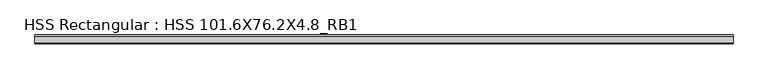
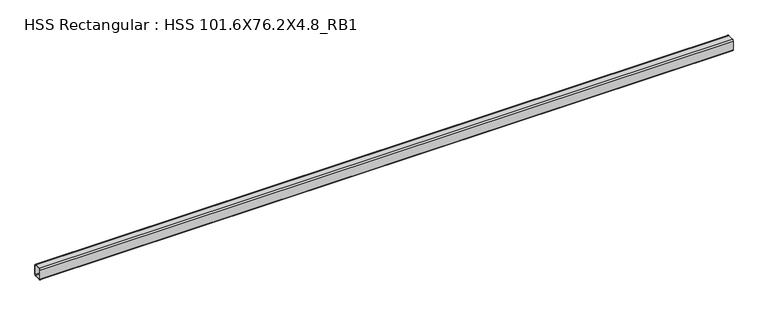
"""IFC4 building model written with IfcOpenShell, lengths in millimetres: beam geometry, HSS Rectangular : HSS 101.6X76.2X4.8_RB1."""

import ifcopenshell
import ifcopenshell.guid

model = None  # the IFC model being written
_history = None  # IfcOwnerHistory: only IFC2X3 demands one
_inside = {}  # id of a spatial element -> (the spatial element, [elements in it])
_under = {}  # id of a project, library or spatial element -> (it, [spatial elements below it])
_declared = {}  # id of a project -> (the project, [libraries it declares])
_typed = {}  # id of a type object -> (the type object, [elements of that type])
_made_of = {}  # id of a material, layer set ... -> (it, [elements and type objects made of it])


def new_model(schema):
    """Start an empty IFC model of exactly this schema.

    Asked for "IFC4X3", IfcOpenShell would pick the latest addendum, in which some entities
    have other attributes; the version numbers below select the first issue.
    IFC2X3 requires an IfcOwnerHistory on every rooted entity: one is made here for all.
    """
    global model, _history
    if schema == "IFC4X3":
        model = ifcopenshell.file(schema_version=(4, 3, 0, 0))
    else:
        model = ifcopenshell.file(schema=schema)
    _inside.clear()
    _under.clear()
    _declared.clear()
    _typed.clear()
    _made_of.clear()
    _history = None
    if model.schema == "IFC2X3":
        org = make("IfcOrganization", Name="unknown")
        user = make(
            "IfcPersonAndOrganization",
            ThePerson=make("IfcPerson", FamilyName="unknown"),
            TheOrganization=org,
        )
        app = make(
            "IfcApplication",
            ApplicationDeveloper=org,
            Version="unknown",
            ApplicationFullName="unknown",
            ApplicationIdentifier="unknown",
        )
        _history = make(
            "IfcOwnerHistory",
            OwningUser=user,
            OwningApplication=app,
            ChangeAction="ADDED",
            CreationDate=0,
        )
    return model


def make(cls, **values):
    """One entity of the class cls with the attributes given. An attribute that is None is left unset."""
    return model.create_entity(
        cls, **{name: value for name, value in values.items() if value is not None}
    )


def rooted(cls, **values):
    """An entity with a GlobalId (a new one), such as an element, a storey or a relation."""
    return make(cls, GlobalId=ifcopenshell.guid.new(), OwnerHistory=_history, **values)


def si_unit(unit_type, name, prefix=None):
    """IfcSIUnit, for example si_unit("LENGTHUNIT", "METRE", prefix="MILLI")."""
    return make("IfcSIUnit", UnitType=unit_type, Prefix=prefix, Name=name)


def assignment(units):
    """IfcUnitAssignment: the units of a project."""
    return None if units is None else make("IfcUnitAssignment", Units=units)


def point(xyz):
    """IfcCartesianPoint."""
    return None if xyz is None else make("IfcCartesianPoint", Coordinates=xyz)


def direction(xyz):
    """IfcDirection."""
    return None if xyz is None else make("IfcDirection", DirectionRatios=xyz)


def frame(location, z_axis=None, x_axis=None):
    """IfcAxis2Placement3D, a coordinate frame: its origin and axes. An axis left out is left unset."""
    return make(
        "IfcAxis2Placement3D",
        Location=point(location),
        Axis=direction(z_axis),
        RefDirection=direction(x_axis),
    )


def frame_2d(location, x_axis=None):
    """IfcAxis2Placement2D, a coordinate frame in the plane: its origin and x axis."""
    return make(
        "IfcAxis2Placement2D", Location=point(location), RefDirection=direction(x_axis)
    )


def origin():
    """The frame at (0, 0, 0) with its axes left unset."""
    return frame((0.0, 0.0, 0.0))


def place(relative_to, where):
    """IfcLocalPlacement: puts the frame where relative to a parent placement (None: the world)."""
    return make(
        "IfcLocalPlacement", PlacementRelTo=relative_to, RelativePlacement=where
    )


def context(
    kind, dimensions, precision=None, world=None, true_north=None, identifier=None
):
    """IfcGeometricRepresentationContext, for example the 3D "Model" context."""
    return make(
        "IfcGeometricRepresentationContext",
        ContextIdentifier=identifier,
        ContextType=kind,
        CoordinateSpaceDimension=dimensions,
        Precision=precision,
        WorldCoordinateSystem=world,
        TrueNorth=true_north,
    )


def project(units=None, contexts=None):
    """IfcProject with its units and contexts."""
    return rooted(
        "IfcProject",
        Name="project",
        RepresentationContexts=contexts,
        UnitsInContext=assignment(units),
    )


def spatial(cls, under=None, at=None, **own):
    """A site, building, storey or space (cls), placed at a placement, below another one or the project."""
    s = rooted(cls, ObjectPlacement=at, **own)
    if under is not None:
        _under.setdefault(under.id(), (under, []))[1].append(s)
    return s


def polyline(points):
    """IfcPolyline through the points."""
    return make("IfcPolyline", Points=[point(p) for p in points])


def circle_curve(where, radius):
    """IfcCircle in the frame where."""
    return make("IfcCircle", Position=where, Radius=radius)


def trimmed(basis, trim1, trim2, sense, master):
    """IfcTrimmedCurve: the piece of a basis curve between two trims."""
    return make(
        "IfcTrimmedCurve",
        BasisCurve=basis,
        Trim1=trim1,
        Trim2=trim2,
        SenseAgreement=sense,
        MasterRepresentation=master,
    )


def segment(curve, same_sense, transition):
    """IfcCompositeCurveSegment."""
    return make(
        "IfcCompositeCurveSegment",
        Transition=transition,
        SameSense=same_sense,
        ParentCurve=curve,
    )


def composite_curve(segments, self_intersect=None):
    """IfcCompositeCurve: segments joined end to end."""
    return make("IfcCompositeCurve", Segments=segments, SelfIntersect=self_intersect)


def outline(outer, holes=None, kind="AREA"):
    """IfcArbitraryClosedProfileDef: a profile drawn as a closed curve; with holes, ...WithVoids."""
    if holes is None:
        return make("IfcArbitraryClosedProfileDef", ProfileType=kind, OuterCurve=outer)
    return make(
        "IfcArbitraryProfileDefWithVoids",
        ProfileType=kind,
        OuterCurve=outer,
        InnerCurves=holes,
    )


def extrude(swept, where, along, depth):
    """IfcExtrudedAreaSolid: the profile swept, set in the frame where, extruded along a direction by depth."""
    return make(
        "IfcExtrudedAreaSolid",
        SweptArea=swept,
        Position=where,
        ExtrudedDirection=direction(along),
        Depth=depth,
    )


def shape(context_of_items, identifier, shape_type, items):
    """IfcShapeRepresentation: the items that make up one representation, for example the "Body"."""
    return make(
        "IfcShapeRepresentation",
        ContextOfItems=context_of_items,
        RepresentationIdentifier=identifier,
        RepresentationType=shape_type,
        Items=items,
    )


def source(mapping_origin, context_of_items, identifier, shape_type, items):
    """IfcRepresentationMap: a shape defined once, which mapped items show again and again."""
    return make(
        "IfcRepresentationMap",
        MappingOrigin=mapping_origin,
        MappedRepresentation=shape(context_of_items, identifier, shape_type, items),
    )


def transform(
    local_origin,
    x_axis=None,
    y_axis=None,
    z_axis=None,
    scale=None,
    scale2=None,
    scale3=None,
    uniform=True,
):
    """IfcCartesianTransformationOperator3D, or its non-uniform kind. x_axis, y_axis, z_axis: its Axis1, 2, 3."""
    if uniform:
        return make(
            "IfcCartesianTransformationOperator3D",
            Axis1=direction(x_axis),
            Axis2=direction(y_axis),
            LocalOrigin=point(local_origin),
            Scale=scale,
            Axis3=direction(z_axis),
        )
    return make(
        "IfcCartesianTransformationOperator3DnonUniform",
        Axis1=direction(x_axis),
        Axis2=direction(y_axis),
        LocalOrigin=point(local_origin),
        Scale=scale,
        Axis3=direction(z_axis),
        Scale2=scale2,
        Scale3=scale3,
    )


def mapped(mapping_source, mapping_target):
    """IfcMappedItem: shows the shape of a source again, moved by a transform."""
    return make(
        "IfcMappedItem", MappingSource=mapping_source, MappingTarget=mapping_target
    )


def made_of(thing, what):
    """Note that an element or type object is made of a material, layer set ...; save() writes the relation."""
    if what is not None:
        _made_of.setdefault(what.id(), (what, []))[1].append(thing)
    return thing


def element(
    cls,
    number,
    at=None,
    inside=None,
    cuts=None,
    type_object=None,
    material=None,
    context=None,
    identifier="Body",
    shape_type=None,
    held_by="IfcProductDefinitionShape",
    body=None,
    shapes=None,
    **own,
):
    """One element of the class cls, such as IfcWall. Its Tag is "e" and its number.

    at: its placement. inside: the storey or other place that contains it. cuts: it is an
    opening in that element (IfcRelVoidsElement). A single representation is given by context,
    identifier, shape_type and body (its items); several are given by shapes. held_by: the class
    of the entity that holds the representations. save() writes the other relations.
    """
    e = rooted(cls, Tag="e%d" % number, ObjectPlacement=at, **own)
    if body is not None:
        shapes = [shape(context, identifier, shape_type, body)]
    if shapes is not None:
        e.Representation = make(held_by, Representations=shapes)
    if inside is not None:
        _inside.setdefault(inside.id(), (inside, []))[1].append(e)
    if cuts is not None:
        rooted(
            "IfcRelVoidsElement", RelatingBuildingElement=cuts, RelatedOpeningElement=e
        )
    if type_object is not None:
        _typed.setdefault(type_object.id(), (type_object, []))[1].append(e)
    return made_of(e, material)


def aggregate(whole, parts):
    """IfcRelAggregates: a whole, such as a stair, and the parts it consists of."""
    return rooted("IfcRelAggregates", RelatingObject=whole, RelatedObjects=parts)


def save(model, path):
    """Write the relations noted so far, then the file.

    IfcRelAggregates (storeys below a building ...), IfcRelContainedInSpatialStructure (elements
    in a storey), IfcRelDefinesByType, IfcRelAssociatesMaterial and IfcRelDeclares: one each for
    every whole, place, type object, material and project.
    """
    for whole, parts in _under.values():
        aggregate(whole, parts)
    for where, things in _inside.values():
        rooted(
            "IfcRelContainedInSpatialStructure",
            RelatedElements=things,
            RelatingStructure=where,
        )
    for kind, things in _typed.values():
        rooted("IfcRelDefinesByType", RelatedObjects=things, RelatingType=kind)
    for what, things in _made_of.values():
        rooted("IfcRelAssociatesMaterial", RelatedObjects=things, RelatingMaterial=what)
    for by, libraries in _declared.values():
        rooted("IfcRelDeclares", RelatingContext=by, RelatedDefinitions=libraries)
    model.write(path)


def hss_rectangular_hss_101_6x76_2x4_8_rb1_b5bc43ef(model_context):
    return source(origin(), model_context, "Body", "SweptSolid", [
        extrude(outline(composite_curve([segment(polyline([(38.1, 41.275), (38.1, -41.275)]), True, "CONTINUOUS"), segment(trimmed(circle_curve(frame_2d((28.575, -41.275)), 9.525), [point((38.1, -41.275))], [point((28.575, -50.8))], False, "CARTESIAN"), True, "CONTINUOUS"), segment(polyline([(28.575, -50.8), (-28.575, -50.8)]), True, "CONTINUOUS"), segment(trimmed(circle_curve(frame_2d((-28.575, -41.275)), 9.525), [point((-28.575, -50.8))], [point((-38.1, -41.275))], False, "CARTESIAN"), True, "CONTINUOUS"), segment(polyline([(-38.1, -41.275), (-38.1, 41.275)]), True, "CONTINUOUS"), segment(trimmed(circle_curve(frame_2d((-28.575, 41.275)), 9.525), [point((-38.1, 41.275))], [point((-28.575, 50.8))], False, "CARTESIAN"), True, "CONTINUOUS"), segment(polyline([(-28.575, 50.8), (28.575, 50.8)]), True, "CONTINUOUS"), segment(trimmed(circle_curve(frame_2d((28.575, 41.275)), 9.525), [point((28.575, 50.8))], [point((38.1, 41.275))], False, "CARTESIAN"), True, "CONTINUOUS")], self_intersect=False), holes=[composite_curve([segment(trimmed(circle_curve(frame_2d((-28.575, 41.275)), 4.7625), [point((-28.575, 46.0375))], [point((-33.3375, 41.275))], True, "CARTESIAN"), True, "CONTINUOUS"), segment(polyline([(-33.3375, 41.275), (-33.3375, -41.275)]), True, "CONTINUOUS"), segment(trimmed(circle_curve(frame_2d((-28.575, -41.275)), 4.7625), [point((-33.3375, -41.275))], [point((-28.575, -46.0375))], True, "CARTESIAN"), True, "CONTINUOUS"), segment(polyline([(-28.575, -46.0375), (28.575, -46.0375)]), True, "CONTINUOUS"), segment(trimmed(circle_curve(frame_2d((28.575, -41.275)), 4.7625), [point((28.575, -46.0375))], [point((33.3375, -41.275))], True, "CARTESIAN"), True, "CONTINUOUS"), segment(polyline([(33.3375, -41.275), (33.3375, 41.275)]), True, "CONTINUOUS"), segment(trimmed(circle_curve(frame_2d((28.575, 41.275)), 4.7625), [point((33.3375, 41.275))], [point((28.575, 46.0375))], True, "CARTESIAN"), True, "CONTINUOUS"), segment(polyline([(28.575, 46.0375), (-28.575, 46.0375)]), True, "CONTINUOUS")], self_intersect=False)]), frame((-7511.1179156, 0.0, 0.0), z_axis=(1.0, 0.0, 0.0), x_axis=(0.0, 1.0, 0.0)), (0.0, 0.0, 1.0), 5998.1692043),
    ])


if __name__ == "__main__":
    model = new_model("IFC4")
    model_context = context("Model", 3, world=origin())
    ifc_project = project(units=[si_unit("LENGTHUNIT", "METRE", prefix="MILLI")], contexts=[model_context])
    site = spatial("IfcSite", under=ifc_project)
    building = spatial("IfcBuilding", under=site)
    placement = place(None, origin())
    hss_rectangular_hss_101_6x76_2x4_8_rb1_shape = hss_rectangular_hss_101_6x76_2x4_8_rb1_b5bc43ef(model_context)
    element("IfcBeam", 1, ObjectType="HSS Rectangular : HSS 101.6X76.2X4.8_RB1", at=placement, inside=building, context=model_context, shape_type="MappedRepresentation", body=[
        mapped(hss_rectangular_hss_101_6x76_2x4_8_rb1_shape, transform((0.0, 0.0, 0.0), x_axis=(1.0, 0.0, 0.0), y_axis=(0.0, 1.0, 0.0), z_axis=(0.0, 0.0, 1.0))),
    ])
    save(model, "model.ifc")

# Revit data of these elements
# Type "HSS Rectangular : HSS 101.6X76.2X4.8_RB1"
#   Section Name Key = "HSS 4X3X3/16"
#   Assembly Code = "B10"
#   Width = 7.62 cm
#   Wall Nominal Thickness = 0.4763 cm
#   Wall Design Thickness = 0.442 cm
#   Torsional Moment of Inertia = 260.561 cm⁴
#   Torsional Modulus = 61.2876 cm³
#   Section Area = 14.4516 cm²
#   Plastic Modulus weak axis = 40.3122 cm³
#   Plastic Modulus strong axis = 49.1612 cm³
#   Perimeter = 0.881482 m²/m
#   Outer Fillet = 0.9525 cm
#   Nominal Weight = 12.1285 kgf/m
#   Moment of Inertia weak axis = 131.529 cm⁴
#   Moment of Inertia strong axis = 205.202 cm⁴
#   Inner Fillet = 0.4763 cm
#   Height = 10.16 cm
#   Elastic Modulus weak axis = 34.4128 cm³
#   Elastic Modulus strong axis = 40.476 cm³
#   Centroid Vertical = 5.08 cm
#   Centroid Horizontal = 3.81 cm
#   Length [instance default] = 1524 mm
#   Structural Material [instance default] = Steel ASTM A500, Grade B, Rectangular and Square
#   Principal Axes Angle = 0
# Element 1 (IfcBeam, "HSS Rectangular : HSS 101.6X76.2X4.8_RB1")
#   Structural Material = Steel ASTM A992
#   Materials on its faces: "Steel ASTM A992"
# Materials
#   "Steel ASTM A500, Grade B, Rectangular and Square": class "Metal", colour RGB 199 199 199, transparency 0, Description = "Carbon steel", Cost = 0
#   "Steel ASTM A992": class "Metal", colour RGB 199 199 199, transparency 0, Description = "Structural steel 50ksi", Cost = 0
